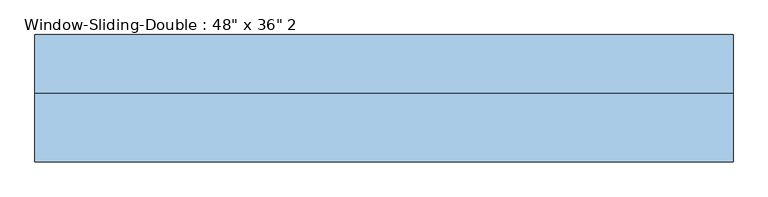
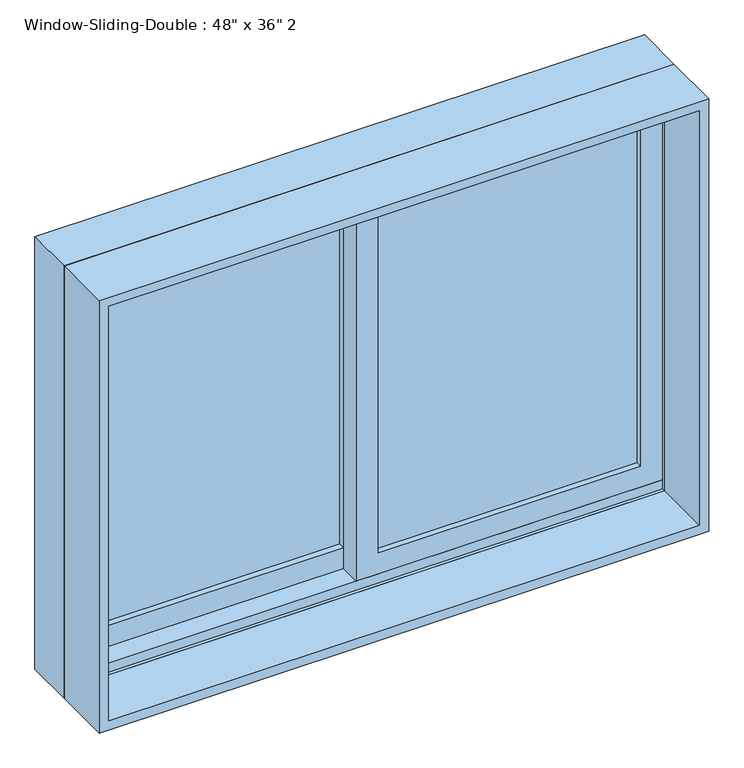
"""IFC4 building model written with IfcOpenShell, lengths in millimetres: window geometry."""

from ifc_helpers import new_model, si_unit, frame, origin, place, context, project, spatial, polyline, outline, extrude, faceted_brep, source, transform, mapped, element, save


def window_3e2df7ed(model_context):
    return source(origin(), model_context, "Body", "SolidModel", [
        faceted_brep([(-609.6, 15.24, 914.4), (-609.6, 116.84, 914.4), (609.6, 116.84, 914.4), (609.6, 15.24, 914.4), (-568.6778905, 116.84, 1787.8778905), (-568.6778905, 110.49, 1787.8778905), (-568.6778905, 110.49, 933.45), (-568.6778905, 116.84, 933.45), (568.6778905, 110.49, 1787.8778905), (568.6778905, 110.49, 933.45), (590.55, 110.49, 933.45), (590.55, 110.49, 1809.75), (-590.55, 110.49, 1809.75), (-590.55, 110.49, 933.45), (-590.55, 15.24, 1809.75), (-590.55, 15.24, 933.45), (-590.55, 21.59, 933.45), (-590.55, 21.59, 952.5), (-590.55, 66.04, 952.5), (-590.55, 66.04, 933.45), (609.6, 15.24, 1828.8), (-609.6, 15.24, 1828.8), (590.55, 15.24, 1809.75), (590.55, 15.24, 933.45), (-609.6, 116.84, 1828.8), (609.6, 116.84, 1828.8), (568.6778905, 116.84, 933.45), (568.6778905, 116.84, 1787.8778905), (590.55, 66.04, 933.45), (590.55, 66.04, 952.5), (590.55, 21.59, 952.5), (590.55, 21.59, 933.45)], [[[0, 1, 2, 3]], [[4, 5, 6, 7]], [[5, 8, 9, 10, 11, 12, 13, 6]], [[12, 14, 15, 16, 17, 18, 19, 13]], [[0, 3, 20, 21], [22, 23, 15, 14]], [[24, 1, 0, 21]], [[2, 1, 24, 25], [4, 7, 26, 27]], [[5, 4, 27, 8]], [[12, 11, 22, 14]], [[21, 20, 25, 24]], [[8, 27, 26, 9]], [[22, 11, 10, 28, 29, 30, 31, 23]], [[20, 3, 2, 25]], [[26, 7, 6, 13, 19, 28, 10, 9]], [[28, 19, 18, 29]], [[29, 18, 17, 30]], [[30, 17, 16, 31]], [[15, 23, 31, 16]]]),
        extrude(outline(polyline([(1828.8, -609.6), (914.4, -609.6), (914.4, 609.6), (1828.8, 609.6), (1828.8, -609.6)]), holes=[polyline([(1809.75, 590.55), (933.45, 590.55), (933.45, -590.55), (1809.75, -590.55), (1809.75, 590.55)])]), frame((0.0, -105.41, 0.0), z_axis=(0.0, 1.0, 0.0), x_axis=(0.0, 0.0, 1.0)), (0.0, 0.0, 1.0), 120.65),
        extrude(outline(polyline([(546.1, 53.34), (546.1, 46.99), (22.225, 46.99), (22.225, 53.34), (546.1, 53.34)])), frame((0.0, 0.0, 996.95), z_axis=(0.0, 0.0, 1.0), x_axis=(1.0, 0.0, 0.0)), (0.0, 0.0, 1.0), 768.35),
        extrude(outline(polyline([(546.1, 40.64), (546.1, 34.29), (22.225, 34.29), (22.225, 40.64), (546.1, 40.64)])), frame((0.0, 0.0, 996.95), z_axis=(0.0, 0.0, 1.0), x_axis=(1.0, 0.0, 0.0)), (0.0, 0.0, 1.0), 768.35),
        extrude(outline(polyline([(-22.225, 97.79), (-22.225, 91.44), (-546.1, 91.44), (-546.1, 97.79), (-22.225, 97.79)])), frame((0.0, 0.0, 996.95), z_axis=(0.0, 0.0, 1.0), x_axis=(1.0, 0.0, 0.0)), (0.0, 0.0, 1.0), 768.35),
        extrude(outline(polyline([(-22.225, 85.09), (-22.225, 78.74), (-546.1, 78.74), (-546.1, 85.09), (-22.225, 85.09)])), frame((0.0, 0.0, 996.95), z_axis=(0.0, 0.0, 1.0), x_axis=(1.0, 0.0, 0.0)), (0.0, 0.0, 1.0), 768.35),
        extrude(outline(polyline([(933.45, -590.55), (933.45, 22.225), (1809.75, 22.225), (1809.75, -590.55), (933.45, -590.55)]), holes=[polyline([(1765.3, -22.225), (996.95, -22.225), (996.95, -546.1), (1765.3, -546.1), (1765.3, -22.225)])]), frame((0.0, 66.04, 0.0), z_axis=(0.0, 1.0, 0.0), x_axis=(0.0, 0.0, 1.0)), (0.0, 0.0, 1.0), 44.45),
        extrude(outline(polyline([(952.5, 590.55), (1809.75, 590.55), (1809.75, -22.225), (952.5, -22.225), (952.5, 590.55)]), holes=[polyline([(996.95, 22.225), (1765.3, 22.225), (1765.3, 546.1), (996.95, 546.1), (996.95, 22.225)])]), frame((0.0, 21.59, 0.0), z_axis=(0.0, 1.0, 0.0), x_axis=(0.0, 0.0, 1.0)), (0.0, 0.0, 1.0), 44.45),
    ])


if __name__ == "__main__":
    model = new_model("IFC4")
    model_context = context("Model", 3, world=origin())
    ifc_project = project(units=[si_unit("LENGTHUNIT", "METRE", prefix="MILLI")], contexts=[model_context])
    site = spatial("IfcSite", under=ifc_project)
    building = spatial("IfcBuilding", under=site)
    placement = place(None, origin())
    window_shape = window_3e2df7ed(model_context)
    element("IfcWindow", 1, ObjectType="Window-Sliding-Double : 48\" x 36\" 2", at=placement, inside=building, context=model_context, shape_type="MappedRepresentation", body=[
        mapped(window_shape, transform((0.0, 0.0, 0.0), x_axis=(1.0, 0.0, 0.0), y_axis=(0.0, 1.0, 0.0), z_axis=(0.0, 0.0, 1.0))),
    ])
    save(model, "model.ifc")

# Revit data of these elements
# Type "Window-Sliding-Double : 48\" x 36\" 2"
#   Type Mark = "16"
#   Fire Rating = "0.5h"
#   Assembly Code = "B2020100"
#   Analytic Construction = "Double glazing - domestic"
#   Window Inset [instance default] = 0' - 0"
#   Wall Thickness [instance default] = 0' - 6"
#   Visual Light Transmittance = 0.81
#   Thermal Resistance (R) = 0.319569 (m²·K)/W
#   Solar Heat Gain Coefficient = 0.76
#   Muntin Width = 1' - 8 5/8"
#   Muntin Height = 2' - 6 1/4"
#   Interior Wall Closure [instance default] = 0' - 2 3/4"
#   Heat Transfer Coefficient (U) = 3.12929 W/(m²·K)
#   Frame Extension [instance default] = 0' - 0 1/4"
#   Exterior Wall Closure [instance default] = 0' - 1 1/4"
#   Rough Width = 4' - 0 1/2"
#   Rough Height = 3' - 0 1/2"
#   Height = 3' - 0"
#   Extension Jamb [instance default] = 0' - 2 3/4"
#   Default Sill Height = 3' - 0"
#   Width = 4' - 0"
#   Interior Trim Visibility [instance default] = yes
#   Indicator Visibility [instance default] = yes
#   Exterior Trim Visibility [instance default] = yes
#   Muntin Visibility = no
#   Extension Jamb Visibility [instance default] = yes
#   Muntin Pattern = Muntin Pattern_2x2 : Muntin Pattern_2x2
#   Interior Trim Material = accent 2
#   Interior Trim = Trim-Window-Interior-Flat : Picture Frame
#   Interior Frame Material = accent 2
#   Glass Panel Material = Glass
#   Exterior Trim Material = accent 2
#   Exterior Trim = Trim-Window-Exterior-Flat : with Sill
#   Exterior Frame Material = accent 2
#   Wall Closure = (empty or 0)
# Element 1 (IfcWindow, "Window-Sliding-Double : 48\" x 36\" 2")
#   Wall Thickness = 0' - 8"
#   Extension Jamb = 0' - 4 3/4"
#   Materials on its faces: "accent 2", "Glass"
# Materials
#   "accent 2": class "Wood", colour RGB 80 80 80, transparency 0, Description = "Wood framing, thermal airspace", Cost = 0
#   "Glass": class "Glass", colour RGB 236 240 239, transparency 0.85, Description = "Soda Lime Glass", Cost = 0
